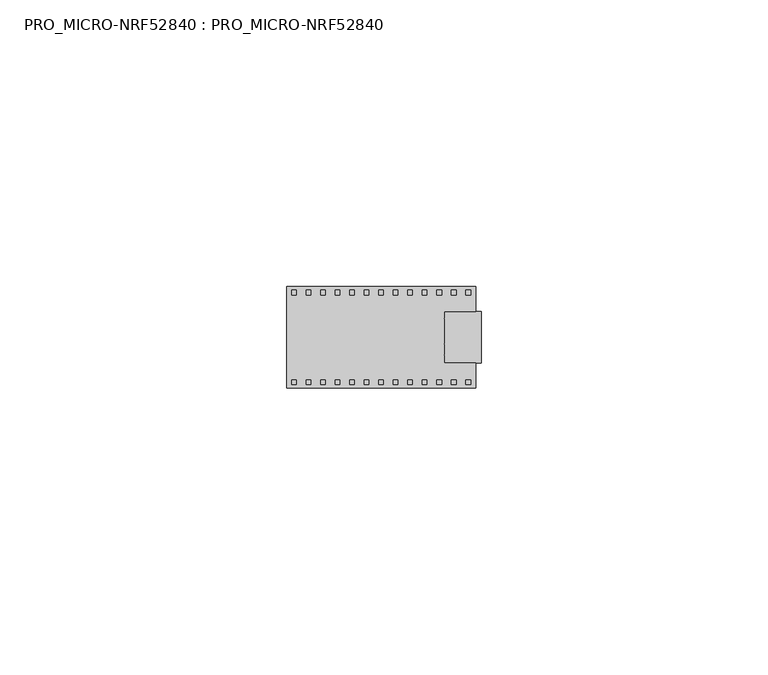
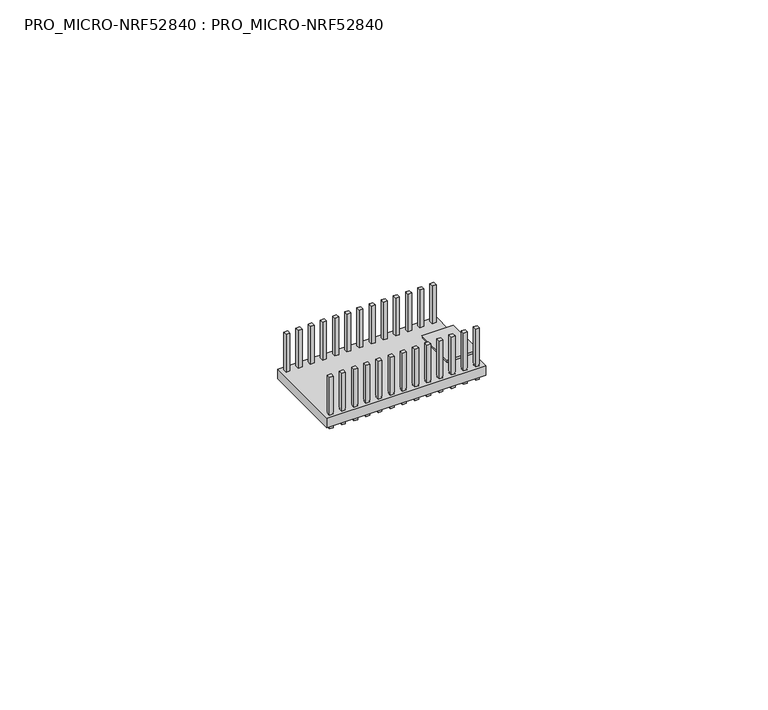
"""IFC4 building model written with IfcOpenShell, lengths in millimetres: furniture geometry, PRO_MICRO-NRF52840 : PRO_MICRO-NRF52840."""

import ifcopenshell
import ifcopenshell.guid

model = None  # the IFC model being written
_history = None  # IfcOwnerHistory: only IFC2X3 demands one
_inside = {}  # id of a spatial element -> (the spatial element, [elements in it])
_under = {}  # id of a project, library or spatial element -> (it, [spatial elements below it])
_declared = {}  # id of a project -> (the project, [libraries it declares])
_typed = {}  # id of a type object -> (the type object, [elements of that type])
_made_of = {}  # id of a material, layer set ... -> (it, [elements and type objects made of it])


def new_model(schema):
    """Start an empty IFC model of exactly this schema.

    Asked for "IFC4X3", IfcOpenShell would pick the latest addendum, in which some entities
    have other attributes; the version numbers below select the first issue.
    IFC2X3 requires an IfcOwnerHistory on every rooted entity: one is made here for all.
    """
    global model, _history
    if schema == "IFC4X3":
        model = ifcopenshell.file(schema_version=(4, 3, 0, 0))
    else:
        model = ifcopenshell.file(schema=schema)
    _inside.clear()
    _under.clear()
    _declared.clear()
    _typed.clear()
    _made_of.clear()
    _history = None
    if model.schema == "IFC2X3":
        org = make("IfcOrganization", Name="unknown")
        user = make(
            "IfcPersonAndOrganization",
            ThePerson=make("IfcPerson", FamilyName="unknown"),
            TheOrganization=org,
        )
        app = make(
            "IfcApplication",
            ApplicationDeveloper=org,
            Version="unknown",
            ApplicationFullName="unknown",
            ApplicationIdentifier="unknown",
        )
        _history = make(
            "IfcOwnerHistory",
            OwningUser=user,
            OwningApplication=app,
            ChangeAction="ADDED",
            CreationDate=0,
        )
    return model


def make(cls, **values):
    """One entity of the class cls with the attributes given. An attribute that is None is left unset."""
    return model.create_entity(
        cls, **{name: value for name, value in values.items() if value is not None}
    )


def rooted(cls, **values):
    """An entity with a GlobalId (a new one), such as an element, a storey or a relation."""
    return make(cls, GlobalId=ifcopenshell.guid.new(), OwnerHistory=_history, **values)


def si_unit(unit_type, name, prefix=None):
    """IfcSIUnit, for example si_unit("LENGTHUNIT", "METRE", prefix="MILLI")."""
    return make("IfcSIUnit", UnitType=unit_type, Prefix=prefix, Name=name)


def assignment(units):
    """IfcUnitAssignment: the units of a project."""
    return None if units is None else make("IfcUnitAssignment", Units=units)


def point(xyz):
    """IfcCartesianPoint."""
    return None if xyz is None else make("IfcCartesianPoint", Coordinates=xyz)


def direction(xyz):
    """IfcDirection."""
    return None if xyz is None else make("IfcDirection", DirectionRatios=xyz)


def frame(location, z_axis=None, x_axis=None):
    """IfcAxis2Placement3D, a coordinate frame: its origin and axes. An axis left out is left unset."""
    return make(
        "IfcAxis2Placement3D",
        Location=point(location),
        Axis=direction(z_axis),
        RefDirection=direction(x_axis),
    )


def origin():
    """The frame at (0, 0, 0) with its axes left unset."""
    return frame((0.0, 0.0, 0.0))


def place(relative_to, where):
    """IfcLocalPlacement: puts the frame where relative to a parent placement (None: the world)."""
    return make(
        "IfcLocalPlacement", PlacementRelTo=relative_to, RelativePlacement=where
    )


def context(
    kind, dimensions, precision=None, world=None, true_north=None, identifier=None
):
    """IfcGeometricRepresentationContext, for example the 3D "Model" context."""
    return make(
        "IfcGeometricRepresentationContext",
        ContextIdentifier=identifier,
        ContextType=kind,
        CoordinateSpaceDimension=dimensions,
        Precision=precision,
        WorldCoordinateSystem=world,
        TrueNorth=true_north,
    )


def project(units=None, contexts=None):
    """IfcProject with its units and contexts."""
    return rooted(
        "IfcProject",
        Name="project",
        RepresentationContexts=contexts,
        UnitsInContext=assignment(units),
    )


def spatial(cls, under=None, at=None, **own):
    """A site, building, storey or space (cls), placed at a placement, below another one or the project."""
    s = rooted(cls, ObjectPlacement=at, **own)
    if under is not None:
        _under.setdefault(under.id(), (under, []))[1].append(s)
    return s


def faces_of(points, faces, orient=None, outer=None):
    """IfcFace entities. A face is a list of loops; a loop is a list of indices into points, from 0.

    orient and outer hold one flag for each loop. By default every Orientation is true, the
    first loop of a face is its IfcFaceOuterBound and the others are IfcFaceBound.
    """
    made = []
    for i, loops in enumerate(faces):
        bounds = []
        for j, loop in enumerate(loops):
            is_outer = j == 0 if outer is None else outer[i][j]
            bounds.append(
                make(
                    "IfcFaceOuterBound" if is_outer else "IfcFaceBound",
                    Bound=make("IfcPolyLoop", Polygon=[points[k] for k in loop]),
                    Orientation=True if orient is None else orient[i][j],
                )
            )
        made.append(make("IfcFace", Bounds=bounds))
    return made


def faceted_brep(points, faces, orient=None, outer=None, voids=None):
    """IfcFacetedBrep: a solid bounded by flat faces; with voids (closed shells), ...WithVoids."""
    shared = [point(p) for p in points]
    hull = make("IfcClosedShell", CfsFaces=faces_of(shared, faces, orient, outer))
    if voids is None:
        return make("IfcFacetedBrep", Outer=hull)
    return make(
        "IfcFacetedBrepWithVoids",
        Outer=hull,
        Voids=[
            make(cls, CfsFaces=faces_of(shared, fs, o, b)) for cls, fs, o, b in voids
        ],
    )


def shape(context_of_items, identifier, shape_type, items):
    """IfcShapeRepresentation: the items that make up one representation, for example the "Body"."""
    return make(
        "IfcShapeRepresentation",
        ContextOfItems=context_of_items,
        RepresentationIdentifier=identifier,
        RepresentationType=shape_type,
        Items=items,
    )


def source(mapping_origin, context_of_items, identifier, shape_type, items):
    """IfcRepresentationMap: a shape defined once, which mapped items show again and again."""
    return make(
        "IfcRepresentationMap",
        MappingOrigin=mapping_origin,
        MappedRepresentation=shape(context_of_items, identifier, shape_type, items),
    )


def transform(
    local_origin,
    x_axis=None,
    y_axis=None,
    z_axis=None,
    scale=None,
    scale2=None,
    scale3=None,
    uniform=True,
):
    """IfcCartesianTransformationOperator3D, or its non-uniform kind. x_axis, y_axis, z_axis: its Axis1, 2, 3."""
    if uniform:
        return make(
            "IfcCartesianTransformationOperator3D",
            Axis1=direction(x_axis),
            Axis2=direction(y_axis),
            LocalOrigin=point(local_origin),
            Scale=scale,
            Axis3=direction(z_axis),
        )
    return make(
        "IfcCartesianTransformationOperator3DnonUniform",
        Axis1=direction(x_axis),
        Axis2=direction(y_axis),
        LocalOrigin=point(local_origin),
        Scale=scale,
        Axis3=direction(z_axis),
        Scale2=scale2,
        Scale3=scale3,
    )


def mapped(mapping_source, mapping_target):
    """IfcMappedItem: shows the shape of a source again, moved by a transform."""
    return make(
        "IfcMappedItem", MappingSource=mapping_source, MappingTarget=mapping_target
    )


def made_of(thing, what):
    """Note that an element or type object is made of a material, layer set ...; save() writes the relation."""
    if what is not None:
        _made_of.setdefault(what.id(), (what, []))[1].append(thing)
    return thing


def element(
    cls,
    number,
    at=None,
    inside=None,
    cuts=None,
    type_object=None,
    material=None,
    context=None,
    identifier="Body",
    shape_type=None,
    held_by="IfcProductDefinitionShape",
    body=None,
    shapes=None,
    **own,
):
    """One element of the class cls, such as IfcWall. Its Tag is "e" and its number.

    at: its placement. inside: the storey or other place that contains it. cuts: it is an
    opening in that element (IfcRelVoidsElement). A single representation is given by context,
    identifier, shape_type and body (its items); several are given by shapes. held_by: the class
    of the entity that holds the representations. save() writes the other relations.
    """
    e = rooted(cls, Tag="e%d" % number, ObjectPlacement=at, **own)
    if body is not None:
        shapes = [shape(context, identifier, shape_type, body)]
    if shapes is not None:
        e.Representation = make(held_by, Representations=shapes)
    if inside is not None:
        _inside.setdefault(inside.id(), (inside, []))[1].append(e)
    if cuts is not None:
        rooted(
            "IfcRelVoidsElement", RelatingBuildingElement=cuts, RelatedOpeningElement=e
        )
    if type_object is not None:
        _typed.setdefault(type_object.id(), (type_object, []))[1].append(e)
    return made_of(e, material)


def aggregate(whole, parts):
    """IfcRelAggregates: a whole, such as a stair, and the parts it consists of."""
    return rooted("IfcRelAggregates", RelatingObject=whole, RelatedObjects=parts)


def save(model, path):
    """Write the relations noted so far, then the file.

    IfcRelAggregates (storeys below a building ...), IfcRelContainedInSpatialStructure (elements
    in a storey), IfcRelDefinesByType, IfcRelAssociatesMaterial and IfcRelDeclares: one each for
    every whole, place, type object, material and project.
    """
    for whole, parts in _under.values():
        aggregate(whole, parts)
    for where, things in _inside.values():
        rooted(
            "IfcRelContainedInSpatialStructure",
            RelatedElements=things,
            RelatingStructure=where,
        )
    for kind, things in _typed.values():
        rooted("IfcRelDefinesByType", RelatedObjects=things, RelatingType=kind)
    for what, things in _made_of.values():
        rooted("IfcRelAssociatesMaterial", RelatedObjects=things, RelatingMaterial=what)
    for by, libraries in _declared.values():
        rooted("IfcRelDeclares", RelatingContext=by, RelatedDefinitions=libraries)
    model.write(path)


def pro_micro_nrf52840_pro_micro_nrf52840_bcfd0b97(model_context):
    return source(origin(), model_context, "Body", "Brep", [
        faceted_brep([(-14.8, 8.2144911, 11.3), (-15.6, 8.2144911, 11.3), (-15.6, 7.4144911, 11.3), (-14.8, 7.4144911, 11.3), (15.6, 8.2144911, 11.3), (14.8, 8.2144911, 11.3), (14.8, 7.4144911, 11.3), (15.6, 7.4144911, 11.3), (13.0666667, 8.2144911, 11.3), (12.2666667, 8.2144911, 11.3), (12.2666667, 7.4144911, 11.3), (13.0666667, 7.4144911, 11.3), (10.5333333, 8.2144911, 11.3), (9.7333333, 8.2144911, 11.3), (9.7333333, 7.4144911, 11.3), (10.5333333, 7.4144911, 11.3), (8.0, 8.2144911, 11.3), (7.2, 8.2144911, 11.3), (7.2, 7.4144911, 11.3), (8.0, 7.4144911, 11.3), (5.4666667, 8.2144911, 11.3), (4.6666667, 8.2144911, 11.3), (4.6666667, 7.4144911, 11.3), (5.4666667, 7.4144911, 11.3), (2.9333333, 8.2144911, 11.3), (2.1333333, 8.2144911, 11.3), (2.1333333, 7.4144911, 11.3), (2.9333333, 7.4144911, 11.3), (0.4, 8.2144911, 11.3), (-0.4, 8.2144911, 11.3), (-0.4, 7.4144911, 11.3), (0.4, 7.4144911, 11.3), (-2.1333333, 8.2144911, 11.3), (-2.9333333, 8.2144911, 11.3), (-2.9333333, 7.4144911, 11.3), (-2.1333333, 7.4144911, 11.3), (-4.6666667, 8.2144911, 11.3), (-5.4666667, 8.2144911, 11.3), (-5.4666667, 7.4144911, 11.3), (-4.6666667, 7.4144911, 11.3), (-7.2, 8.2144911, 11.3), (-8.0, 8.2144911, 11.3), (-8.0, 7.4144911, 11.3), (-7.2, 7.4144911, 11.3), (-9.7333333, 8.2144911, 11.3), (-10.5333333, 8.2144911, 11.3), (-10.5333333, 7.4144911, 11.3), (-9.7333333, 7.4144911, 11.3), (-12.2666667, 8.2144911, 11.3), (-13.0666667, 8.2144911, 11.3), (-13.0666667, 7.4144911, 11.3), (-12.2666667, 7.4144911, 11.3), (-14.8, 8.2144911, 0.0), (-14.8, 7.4144911, 0.0), (-15.6, 7.4144911, 0.0), (-15.6, 8.2144911, 0.0), (15.6, 8.2144911, 0.0), (15.6, 7.4144911, 0.0), (14.8, 7.4144911, 0.0), (14.8, 8.2144911, 0.0), (13.0666667, 8.2144911, 0.0), (13.0666667, 7.4144911, 0.0), (12.2666667, 7.4144911, 0.0), (12.2666667, 8.2144911, 0.0), (10.5333333, 8.2144911, 0.0), (10.5333333, 7.4144911, 0.0), (9.7333333, 7.4144911, 0.0), (9.7333333, 8.2144911, 0.0), (8.0, 8.2144911, 0.0), (8.0, 7.4144911, 0.0), (7.2, 7.4144911, 0.0), (7.2, 8.2144911, 0.0), (5.4666667, 8.2144911, 0.0), (5.4666667, 7.4144911, 0.0), (4.6666667, 7.4144911, 0.0), (4.6666667, 8.2144911, 0.0), (2.9333333, 8.2144911, 0.0), (2.9333333, 7.4144911, 0.0), (2.1333333, 7.4144911, 0.0), (2.1333333, 8.2144911, 0.0), (0.4, 8.2144911, 0.0), (0.4, 7.4144911, 0.0), (-0.4, 7.4144911, 0.0), (-0.4, 8.2144911, 0.0), (-2.1333333, 8.2144911, 0.0), (-2.1333333, 7.4144911, 0.0), (-2.9333333, 7.4144911, 0.0), (-2.9333333, 8.2144911, 0.0), (-4.6666667, 8.2144911, 0.0), (-4.6666667, 7.4144911, 0.0), (-5.4666667, 7.4144911, 0.0), (-5.4666667, 8.2144911, 0.0), (-7.2, 8.2144911, 0.0), (-7.2, 7.4144911, 0.0), (-8.0, 7.4144911, 0.0), (-8.0, 8.2144911, 0.0), (-9.7333333, 8.2144911, 0.0), (-9.7333333, 7.4144911, 0.0), (-10.5333333, 7.4144911, 0.0), (-10.5333333, 8.2144911, 0.0), (-12.2666667, 8.2144911, 0.0), (-12.2666667, 7.4144911, 0.0), (-13.0666667, 7.4144911, 0.0), (-13.0666667, 8.2144911, 0.0), (-14.8, 8.2144911, 3.0), (-15.6, 8.2144911, 3.0), (-15.6, 8.2144911, 1.0), (-14.8, 8.2144911, 1.0), (-15.6, 7.4144911, 3.0), (-15.6, 7.4144911, 1.0), (-14.8, 7.4144911, 3.0), (-14.8, 7.4144911, 1.0), (15.6, 8.2144911, 3.0), (14.8, 8.2144911, 3.0), (14.8, 8.2144911, 1.0), (15.6, 8.2144911, 1.0), (14.8, 7.4144911, 3.0), (14.8, 7.4144911, 1.0), (15.6, 7.4144911, 3.0), (15.6, 7.4144911, 1.0), (13.0666667, 8.2144911, 3.0), (12.2666667, 8.2144911, 3.0), (12.2666667, 8.2144911, 1.0), (13.0666667, 8.2144911, 1.0), (12.2666667, 7.4144911, 3.0), (12.2666667, 7.4144911, 1.0), (13.0666667, 7.4144911, 3.0), (13.0666667, 7.4144911, 1.0), (10.5333333, 8.2144911, 3.0), (9.7333333, 8.2144911, 3.0), (9.7333333, 8.2144911, 1.0), (10.5333333, 8.2144911, 1.0), (9.7333333, 7.4144911, 3.0), (9.7333333, 7.4144911, 1.0), (10.5333333, 7.4144911, 3.0), (10.5333333, 7.4144911, 1.0), (8.0, 8.2144911, 3.0), (7.2, 8.2144911, 3.0), (7.2, 8.2144911, 1.0), (8.0, 8.2144911, 1.0), (7.2, 7.4144911, 3.0), (7.2, 7.4144911, 1.0), (8.0, 7.4144911, 3.0), (8.0, 7.4144911, 1.0), (5.4666667, 8.2144911, 3.0), (4.6666667, 8.2144911, 3.0), (4.6666667, 8.2144911, 1.0), (5.4666667, 8.2144911, 1.0), (4.6666667, 7.4144911, 3.0), (4.6666667, 7.4144911, 1.0), (5.4666667, 7.4144911, 3.0), (5.4666667, 7.4144911, 1.0), (2.9333333, 8.2144911, 3.0), (2.1333333, 8.2144911, 3.0), (2.1333333, 8.2144911, 1.0), (2.9333333, 8.2144911, 1.0), (2.1333333, 7.4144911, 3.0), (2.1333333, 7.4144911, 1.0), (2.9333333, 7.4144911, 3.0), (2.9333333, 7.4144911, 1.0), (0.4, 8.2144911, 3.0), (-0.4, 8.2144911, 3.0), (-0.4, 8.2144911, 1.0), (0.4, 8.2144911, 1.0), (-0.4, 7.4144911, 3.0), (-0.4, 7.4144911, 1.0), (0.4, 7.4144911, 3.0), (0.4, 7.4144911, 1.0), (-2.1333333, 8.2144911, 3.0), (-2.9333333, 8.2144911, 3.0), (-2.9333333, 8.2144911, 1.0), (-2.1333333, 8.2144911, 1.0), (-2.9333333, 7.4144911, 3.0), (-2.9333333, 7.4144911, 1.0), (-2.1333333, 7.4144911, 3.0), (-2.1333333, 7.4144911, 1.0), (-4.6666667, 8.2144911, 3.0), (-5.4666667, 8.2144911, 3.0), (-5.4666667, 8.2144911, 1.0), (-4.6666667, 8.2144911, 1.0), (-5.4666667, 7.4144911, 3.0), (-5.4666667, 7.4144911, 1.0), (-4.6666667, 7.4144911, 3.0), (-4.6666667, 7.4144911, 1.0), (-7.2, 8.2144911, 3.0), (-8.0, 8.2144911, 3.0), (-8.0, 8.2144911, 1.0), (-7.2, 8.2144911, 1.0), (-8.0, 7.4144911, 3.0), (-8.0, 7.4144911, 1.0), (-7.2, 7.4144911, 3.0), (-7.2, 7.4144911, 1.0), (-9.7333333, 8.2144911, 3.0), (-10.5333333, 8.2144911, 3.0), (-10.5333333, 8.2144911, 1.0), (-9.7333333, 8.2144911, 1.0), (-10.5333333, 7.4144911, 3.0), (-10.5333333, 7.4144911, 1.0), (-9.7333333, 7.4144911, 3.0), (-9.7333333, 7.4144911, 1.0), (-12.2666667, 8.2144911, 3.0), (-13.0666667, 8.2144911, 3.0), (-13.0666667, 8.2144911, 1.0), (-12.2666667, 8.2144911, 1.0), (-13.0666667, 7.4144911, 3.0), (-13.0666667, 7.4144911, 1.0), (-12.2666667, 7.4144911, 3.0), (-12.2666667, 7.4144911, 1.0), (16.5, 8.89, 3.0), (-16.5, 8.89, 3.0), (-16.5, -8.89, 3.0), (16.5, -8.89, 3.0), (16.5, -4.5, 3.0), (11.0, -4.5, 3.0), (11.0, 4.5, 3.0), (16.5, 4.5, 3.0), (-14.8, -8.2144911, 3.0), (-15.6, -8.2144911, 3.0), (-15.6, -7.4144911, 3.0), (-14.8, -7.4144911, 3.0), (15.6, -8.2144911, 3.0), (14.8, -8.2144911, 3.0), (14.8, -7.4144911, 3.0), (15.6, -7.4144911, 3.0), (13.0666667, -8.2144911, 3.0), (12.2666667, -8.2144911, 3.0), (12.2666667, -7.4144911, 3.0), (13.0666667, -7.4144911, 3.0), (10.5333333, -8.2144911, 3.0), (9.7333333, -8.2144911, 3.0), (9.7333333, -7.4144911, 3.0), (10.5333333, -7.4144911, 3.0), (8.0, -8.2144911, 3.0), (7.2, -8.2144911, 3.0), (7.2, -7.4144911, 3.0), (8.0, -7.4144911, 3.0), (5.4666667, -8.2144911, 3.0), (4.6666667, -8.2144911, 3.0), (4.6666667, -7.4144911, 3.0), (5.4666667, -7.4144911, 3.0), (2.9333333, -8.2144911, 3.0), (2.1333333, -8.2144911, 3.0), (2.1333333, -7.4144911, 3.0), (2.9333333, -7.4144911, 3.0), (0.4, -8.2144911, 3.0), (-0.4, -8.2144911, 3.0), (-0.4, -7.4144911, 3.0), (0.4, -7.4144911, 3.0), (-2.1333333, -8.2144911, 3.0), (-2.9333333, -8.2144911, 3.0), (-2.9333333, -7.4144911, 3.0), (-2.1333333, -7.4144911, 3.0), (-4.6666667, -8.2144911, 3.0), (-5.4666667, -8.2144911, 3.0), (-5.4666667, -7.4144911, 3.0), (-4.6666667, -7.4144911, 3.0), (-7.2, -8.2144911, 3.0), (-8.0, -8.2144911, 3.0), (-8.0, -7.4144911, 3.0), (-7.2, -7.4144911, 3.0), (-9.7333333, -8.2144911, 3.0), (-10.5333333, -8.2144911, 3.0), (-10.5333333, -7.4144911, 3.0), (-9.7333333, -7.4144911, 3.0), (-12.2666667, -8.2144911, 3.0), (-13.0666667, -8.2144911, 3.0), (-13.0666667, -7.4144911, 3.0), (-12.2666667, -7.4144911, 3.0), (16.5, -8.89, 1.0), (-16.5, -8.89, 1.0), (-16.5, 8.89, 1.0), (16.5, 8.89, 1.0), (16.5, 4.5, 1.0), (11.0, 4.5, 1.0), (11.0, -4.5, 1.0), (16.5, -4.5, 1.0), (-15.6, -8.2144911, 1.0), (-14.8, -8.2144911, 1.0), (-14.8, -7.4144911, 1.0), (-15.6, -7.4144911, 1.0), (14.8, -8.2144911, 1.0), (15.6, -8.2144911, 1.0), (15.6, -7.4144911, 1.0), (14.8, -7.4144911, 1.0), (12.2666667, -8.2144911, 1.0), (13.0666667, -8.2144911, 1.0), (13.0666667, -7.4144911, 1.0), (12.2666667, -7.4144911, 1.0), (9.7333333, -8.2144911, 1.0), (10.5333333, -8.2144911, 1.0), (10.5333333, -7.4144911, 1.0), (9.7333333, -7.4144911, 1.0), (7.2, -8.2144911, 1.0), (8.0, -8.2144911, 1.0), (8.0, -7.4144911, 1.0), (7.2, -7.4144911, 1.0), (4.6666667, -8.2144911, 1.0), (5.4666667, -8.2144911, 1.0), (5.4666667, -7.4144911, 1.0), (4.6666667, -7.4144911, 1.0), (2.1333333, -8.2144911, 1.0), (2.9333333, -8.2144911, 1.0), (2.9333333, -7.4144911, 1.0), (2.1333333, -7.4144911, 1.0), (-0.4, -8.2144911, 1.0), (0.4, -8.2144911, 1.0), (0.4, -7.4144911, 1.0), (-0.4, -7.4144911, 1.0), (-2.9333333, -8.2144911, 1.0), (-2.1333333, -8.2144911, 1.0), (-2.1333333, -7.4144911, 1.0), (-2.9333333, -7.4144911, 1.0), (-5.4666667, -8.2144911, 1.0), (-4.6666667, -8.2144911, 1.0), (-4.6666667, -7.4144911, 1.0), (-5.4666667, -7.4144911, 1.0), (-8.0, -8.2144911, 1.0), (-7.2, -8.2144911, 1.0), (-7.2, -7.4144911, 1.0), (-8.0, -7.4144911, 1.0), (-10.5333333, -8.2144911, 1.0), (-9.7333333, -8.2144911, 1.0), (-9.7333333, -7.4144911, 1.0), (-10.5333333, -7.4144911, 1.0), (-13.0666667, -8.2144911, 1.0), (-12.2666667, -8.2144911, 1.0), (-12.2666667, -7.4144911, 1.0), (-13.0666667, -7.4144911, 1.0), (-14.8, -8.2144911, 11.3), (-14.8, -7.4144911, 11.3), (-15.6, -7.4144911, 11.3), (-15.6, -8.2144911, 11.3), (15.6, -8.2144911, 11.3), (15.6, -7.4144911, 11.3), (14.8, -7.4144911, 11.3), (14.8, -8.2144911, 11.3), (13.0666667, -8.2144911, 11.3), (13.0666667, -7.4144911, 11.3), (12.2666667, -7.4144911, 11.3), (12.2666667, -8.2144911, 11.3), (10.5333333, -8.2144911, 11.3), (10.5333333, -7.4144911, 11.3), (9.7333333, -7.4144911, 11.3), (9.7333333, -8.2144911, 11.3), (8.0, -8.2144911, 11.3), (8.0, -7.4144911, 11.3), (7.2, -7.4144911, 11.3), (7.2, -8.2144911, 11.3), (5.4666667, -8.2144911, 11.3), (5.4666667, -7.4144911, 11.3), (4.6666667, -7.4144911, 11.3), (4.6666667, -8.2144911, 11.3), (2.9333333, -8.2144911, 11.3), (2.9333333, -7.4144911, 11.3), (2.1333333, -7.4144911, 11.3), (2.1333333, -8.2144911, 11.3), (0.4, -8.2144911, 11.3), (0.4, -7.4144911, 11.3), (-0.4, -7.4144911, 11.3), (-0.4, -8.2144911, 11.3), (-2.1333333, -8.2144911, 11.3), (-2.1333333, -7.4144911, 11.3), (-2.9333333, -7.4144911, 11.3), (-2.9333333, -8.2144911, 11.3), (-4.6666667, -8.2144911, 11.3), (-4.6666667, -7.4144911, 11.3), (-5.4666667, -7.4144911, 11.3), (-5.4666667, -8.2144911, 11.3), (-7.2, -8.2144911, 11.3), (-7.2, -7.4144911, 11.3), (-8.0, -7.4144911, 11.3), (-8.0, -8.2144911, 11.3), (-9.7333333, -8.2144911, 11.3), (-9.7333333, -7.4144911, 11.3), (-10.5333333, -7.4144911, 11.3), (-10.5333333, -8.2144911, 11.3), (-12.2666667, -8.2144911, 11.3), (-12.2666667, -7.4144911, 11.3), (-13.0666667, -7.4144911, 11.3), (-13.0666667, -8.2144911, 11.3), (-14.8, -8.2144911, 0.0), (-15.6, -8.2144911, 0.0), (-15.6, -7.4144911, 0.0), (-14.8, -7.4144911, 0.0), (15.6, -8.2144911, 0.0), (14.8, -8.2144911, 0.0), (14.8, -7.4144911, 0.0), (15.6, -7.4144911, 0.0), (13.0666667, -8.2144911, 0.0), (12.2666667, -8.2144911, 0.0), (12.2666667, -7.4144911, 0.0), (13.0666667, -7.4144911, 0.0), (10.5333333, -8.2144911, 0.0), (9.7333333, -8.2144911, 0.0), (9.7333333, -7.4144911, 0.0), (10.5333333, -7.4144911, 0.0), (8.0, -8.2144911, 0.0), (7.2, -8.2144911, 0.0), (7.2, -7.4144911, 0.0), (8.0, -7.4144911, 0.0), (5.4666667, -8.2144911, 0.0), (4.6666667, -8.2144911, 0.0), (4.6666667, -7.4144911, 0.0), (5.4666667, -7.4144911, 0.0), (2.9333333, -8.2144911, 0.0), (2.1333333, -8.2144911, 0.0), (2.1333333, -7.4144911, 0.0), (2.9333333, -7.4144911, 0.0), (0.4, -8.2144911, 0.0), (-0.4, -8.2144911, 0.0), (-0.4, -7.4144911, 0.0), (0.4, -7.4144911, 0.0), (-2.1333333, -8.2144911, 0.0), (-2.9333333, -8.2144911, 0.0), (-2.9333333, -7.4144911, 0.0), (-2.1333333, -7.4144911, 0.0), (-4.6666667, -8.2144911, 0.0), (-5.4666667, -8.2144911, 0.0), (-5.4666667, -7.4144911, 0.0), (-4.6666667, -7.4144911, 0.0), (-7.2, -8.2144911, 0.0), (-8.0, -8.2144911, 0.0), (-8.0, -7.4144911, 0.0), (-7.2, -7.4144911, 0.0), (-9.7333333, -8.2144911, 0.0), (-10.5333333, -8.2144911, 0.0), (-10.5333333, -7.4144911, 0.0), (-9.7333333, -7.4144911, 0.0), (-12.2666667, -8.2144911, 0.0), (-13.0666667, -8.2144911, 0.0), (-13.0666667, -7.4144911, 0.0), (-12.2666667, -7.4144911, 0.0), (11.0, 4.5, 3.5), (11.0, -4.5, 3.5), (17.5, -4.5, 3.5), (17.5, 4.5, 3.5), (11.0, 4.5, 0.0), (17.5, 4.5, 0.0), (17.5, -4.5, 0.0), (11.0, -4.5, 0.0)], [[[0, 1, 2, 3]], [[4, 5, 6, 7]], [[8, 9, 10, 11]], [[12, 13, 14, 15]], [[16, 17, 18, 19]], [[20, 21, 22, 23]], [[24, 25, 26, 27]], [[28, 29, 30, 31]], [[32, 33, 34, 35]], [[36, 37, 38, 39]], [[40, 41, 42, 43]], [[44, 45, 46, 47]], [[48, 49, 50, 51]], [[52, 53, 54, 55]], [[56, 57, 58, 59]], [[60, 61, 62, 63]], [[64, 65, 66, 67]], [[68, 69, 70, 71]], [[72, 73, 74, 75]], [[76, 77, 78, 79]], [[80, 81, 82, 83]], [[84, 85, 86, 87]], [[88, 89, 90, 91]], [[92, 93, 94, 95]], [[96, 97, 98, 99]], [[100, 101, 102, 103]], [[1, 0, 104, 105]], [[52, 55, 106, 107]], [[2, 1, 105, 108]], [[55, 54, 109, 106]], [[3, 2, 108, 110]], [[54, 53, 111, 109]], [[0, 3, 110, 104]], [[53, 52, 107, 111]], [[5, 4, 112, 113]], [[56, 59, 114, 115]], [[6, 5, 113, 116]], [[59, 58, 117, 114]], [[7, 6, 116, 118]], [[58, 57, 119, 117]], [[4, 7, 118, 112]], [[57, 56, 115, 119]], [[9, 8, 120, 121]], [[60, 63, 122, 123]], [[10, 9, 121, 124]], [[63, 62, 125, 122]], [[11, 10, 124, 126]], [[62, 61, 127, 125]], [[8, 11, 126, 120]], [[61, 60, 123, 127]], [[13, 12, 128, 129]], [[64, 67, 130, 131]], [[14, 13, 129, 132]], [[67, 66, 133, 130]], [[15, 14, 132, 134]], [[66, 65, 135, 133]], [[12, 15, 134, 128]], [[65, 64, 131, 135]], [[17, 16, 136, 137]], [[68, 71, 138, 139]], [[18, 17, 137, 140]], [[71, 70, 141, 138]], [[19, 18, 140, 142]], [[70, 69, 143, 141]], [[16, 19, 142, 136]], [[69, 68, 139, 143]], [[21, 20, 144, 145]], [[72, 75, 146, 147]], [[22, 21, 145, 148]], [[75, 74, 149, 146]], [[23, 22, 148, 150]], [[74, 73, 151, 149]], [[20, 23, 150, 144]], [[73, 72, 147, 151]], [[25, 24, 152, 153]], [[76, 79, 154, 155]], [[26, 25, 153, 156]], [[79, 78, 157, 154]], [[27, 26, 156, 158]], [[78, 77, 159, 157]], [[24, 27, 158, 152]], [[77, 76, 155, 159]], [[29, 28, 160, 161]], [[80, 83, 162, 163]], [[30, 29, 161, 164]], [[83, 82, 165, 162]], [[31, 30, 164, 166]], [[82, 81, 167, 165]], [[28, 31, 166, 160]], [[81, 80, 163, 167]], [[33, 32, 168, 169]], [[84, 87, 170, 171]], [[34, 33, 169, 172]], [[87, 86, 173, 170]], [[35, 34, 172, 174]], [[86, 85, 175, 173]], [[32, 35, 174, 168]], [[85, 84, 171, 175]], [[37, 36, 176, 177]], [[88, 91, 178, 179]], [[38, 37, 177, 180]], [[91, 90, 181, 178]], [[39, 38, 180, 182]], [[90, 89, 183, 181]], [[36, 39, 182, 176]], [[89, 88, 179, 183]], [[41, 40, 184, 185]], [[92, 95, 186, 187]], [[42, 41, 185, 188]], [[95, 94, 189, 186]], [[43, 42, 188, 190]], [[94, 93, 191, 189]], [[40, 43, 190, 184]], [[93, 92, 187, 191]], [[45, 44, 192, 193]], [[96, 99, 194, 195]], [[46, 45, 193, 196]], [[99, 98, 197, 194]], [[47, 46, 196, 198]], [[98, 97, 199, 197]], [[44, 47, 198, 192]], [[97, 96, 195, 199]], [[49, 48, 200, 201]], [[100, 103, 202, 203]], [[50, 49, 201, 204]], [[103, 102, 205, 202]], [[51, 50, 204, 206]], [[102, 101, 207, 205]], [[48, 51, 206, 200]], [[101, 100, 203, 207]], [[208, 209, 210, 211, 212, 213, 214, 215], [105, 104, 110, 108], [113, 112, 118, 116], [121, 120, 126, 124], [129, 128, 134, 132], [137, 136, 142, 140], [145, 144, 150, 148], [153, 152, 158, 156], [161, 160, 166, 164], [169, 168, 174, 172], [177, 176, 182, 180], [185, 184, 190, 188], [193, 192, 198, 196], [201, 200, 206, 204], [216, 217, 218, 219], [220, 221, 222, 223], [224, 225, 226, 227], [228, 229, 230, 231], [232, 233, 234, 235], [236, 237, 238, 239], [240, 241, 242, 243], [244, 245, 246, 247], [248, 249, 250, 251], [252, 253, 254, 255], [256, 257, 258, 259], [260, 261, 262, 263], [264, 265, 266, 267]], [[268, 269, 270, 271, 272, 273, 274, 275], [107, 106, 109, 111], [115, 114, 117, 119], [123, 122, 125, 127], [131, 130, 133, 135], [139, 138, 141, 143], [147, 146, 149, 151], [155, 154, 157, 159], [163, 162, 165, 167], [171, 170, 173, 175], [179, 178, 181, 183], [187, 186, 189, 191], [195, 194, 197, 199], [203, 202, 205, 207], [276, 277, 278, 279], [280, 281, 282, 283], [284, 285, 286, 287], [288, 289, 290, 291], [292, 293, 294, 295], [296, 297, 298, 299], [300, 301, 302, 303], [304, 305, 306, 307], [308, 309, 310, 311], [312, 313, 314, 315], [316, 317, 318, 319], [320, 321, 322, 323], [324, 325, 326, 327]], [[209, 208, 271, 270]], [[210, 209, 270, 269]], [[211, 210, 269, 268]], [[271, 208, 215, 272]], [[211, 268, 275, 212]], [[328, 329, 330, 331]], [[332, 333, 334, 335]], [[336, 337, 338, 339]], [[340, 341, 342, 343]], [[344, 345, 346, 347]], [[348, 349, 350, 351]], [[352, 353, 354, 355]], [[356, 357, 358, 359]], [[360, 361, 362, 363]], [[364, 365, 366, 367]], [[368, 369, 370, 371]], [[372, 373, 374, 375]], [[376, 377, 378, 379]], [[380, 381, 382, 383]], [[384, 385, 386, 387]], [[388, 389, 390, 391]], [[392, 393, 394, 395]], [[396, 397, 398, 399]], [[400, 401, 402, 403]], [[404, 405, 406, 407]], [[408, 409, 410, 411]], [[412, 413, 414, 415]], [[416, 417, 418, 419]], [[420, 421, 422, 423]], [[424, 425, 426, 427]], [[428, 429, 430, 431]], [[328, 331, 217, 216]], [[381, 380, 277, 276]], [[331, 330, 218, 217]], [[382, 381, 276, 279]], [[330, 329, 219, 218]], [[383, 382, 279, 278]], [[329, 328, 216, 219]], [[380, 383, 278, 277]], [[332, 335, 221, 220]], [[385, 384, 281, 280]], [[335, 334, 222, 221]], [[386, 385, 280, 283]], [[334, 333, 223, 222]], [[387, 386, 283, 282]], [[333, 332, 220, 223]], [[384, 387, 282, 281]], [[336, 339, 225, 224]], [[389, 388, 285, 284]], [[339, 338, 226, 225]], [[390, 389, 284, 287]], [[338, 337, 227, 226]], [[391, 390, 287, 286]], [[337, 336, 224, 227]], [[388, 391, 286, 285]], [[340, 343, 229, 228]], [[393, 392, 289, 288]], [[343, 342, 230, 229]], [[394, 393, 288, 291]], [[342, 341, 231, 230]], [[395, 394, 291, 290]], [[341, 340, 228, 231]], [[392, 395, 290, 289]], [[344, 347, 233, 232]], [[397, 396, 293, 292]], [[347, 346, 234, 233]], [[398, 397, 292, 295]], [[346, 345, 235, 234]], [[399, 398, 295, 294]], [[345, 344, 232, 235]], [[396, 399, 294, 293]], [[348, 351, 237, 236]], [[401, 400, 297, 296]], [[351, 350, 238, 237]], [[402, 401, 296, 299]], [[350, 349, 239, 238]], [[403, 402, 299, 298]], [[349, 348, 236, 239]], [[400, 403, 298, 297]], [[352, 355, 241, 240]], [[405, 404, 301, 300]], [[355, 354, 242, 241]], [[406, 405, 300, 303]], [[354, 353, 243, 242]], [[407, 406, 303, 302]], [[353, 352, 240, 243]], [[404, 407, 302, 301]], [[356, 359, 245, 244]], [[409, 408, 305, 304]], [[359, 358, 246, 245]], [[410, 409, 304, 307]], [[358, 357, 247, 246]], [[411, 410, 307, 306]], [[357, 356, 244, 247]], [[408, 411, 306, 305]], [[360, 363, 249, 248]], [[413, 412, 309, 308]], [[363, 362, 250, 249]], [[414, 413, 308, 311]], [[362, 361, 251, 250]], [[415, 414, 311, 310]], [[361, 360, 248, 251]], [[412, 415, 310, 309]], [[364, 367, 253, 252]], [[417, 416, 313, 312]], [[367, 366, 254, 253]], [[418, 417, 312, 315]], [[366, 365, 255, 254]], [[419, 418, 315, 314]], [[365, 364, 252, 255]], [[416, 419, 314, 313]], [[368, 371, 257, 256]], [[421, 420, 317, 316]], [[371, 370, 258, 257]], [[422, 421, 316, 319]], [[370, 369, 259, 258]], [[423, 422, 319, 318]], [[369, 368, 256, 259]], [[420, 423, 318, 317]], [[372, 375, 261, 260]], [[425, 424, 321, 320]], [[375, 374, 262, 261]], [[426, 425, 320, 323]], [[374, 373, 263, 262]], [[427, 426, 323, 322]], [[373, 372, 260, 263]], [[424, 427, 322, 321]], [[376, 379, 265, 264]], [[429, 428, 325, 324]], [[379, 378, 266, 265]], [[430, 429, 324, 327]], [[378, 377, 267, 266]], [[431, 430, 327, 326]], [[377, 376, 264, 267]], [[428, 431, 326, 325]], [[432, 433, 434, 435]], [[436, 437, 438, 439]], [[433, 432, 214, 213]], [[436, 439, 274, 273]], [[434, 433, 213, 212, 275, 274, 439, 438]], [[435, 434, 438, 437]], [[432, 435, 437, 436, 273, 272, 215, 214]]]),
    ])


if __name__ == "__main__":
    model = new_model("IFC4")
    model_context = context("Model", 3, world=origin())
    ifc_project = project(units=[si_unit("LENGTHUNIT", "METRE", prefix="MILLI")], contexts=[model_context])
    site = spatial("IfcSite", under=ifc_project)
    building = spatial("IfcBuilding", under=site)
    placement = place(None, origin())
    pro_micro_nrf52840_pro_micro_nrf52840_shape = pro_micro_nrf52840_pro_micro_nrf52840_bcfd0b97(model_context)
    element("IfcFurniture", 1, ObjectType="PRO_MICRO-NRF52840 : PRO_MICRO-NRF52840", at=placement, inside=building, context=model_context, shape_type="MappedRepresentation", body=[
        mapped(pro_micro_nrf52840_pro_micro_nrf52840_shape, transform((0.0, 0.0, 0.0), x_axis=(1.0, 0.0, 0.0), y_axis=(0.0, 1.0, 0.0), z_axis=(0.0, 0.0, 1.0))),
    ])
    save(model, "model.ifc")

# Revit data of these elements
# Project information
#   Data de emissão do projeto = "Data de emissão"
#   Status do projeto = "Status do projeto"
#   Nome do cliente = "Proprietário"
#   Endereço do projeto = "Insira aqui o endereço"
#   Nome do projeto = "Nome do projeto"
#   Número do projeto = "0001"
# Type "PRO_MICRO-NRF52840 : PRO_MICRO-NRF52840"
#   Default Elevation = 0
# Element 1 (IfcFurniture, "PRO_MICRO-NRF52840 : PRO_MICRO-NRF52840")
#   Materials on its faces: ".CHIP"
# Materials
#   ".CHIP": class "Vidro", colour RGB 236 240 239, transparency 0.35, Cost = 0
